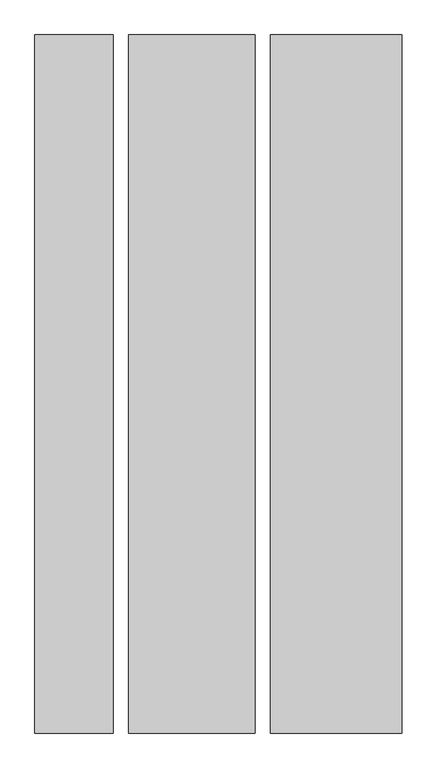
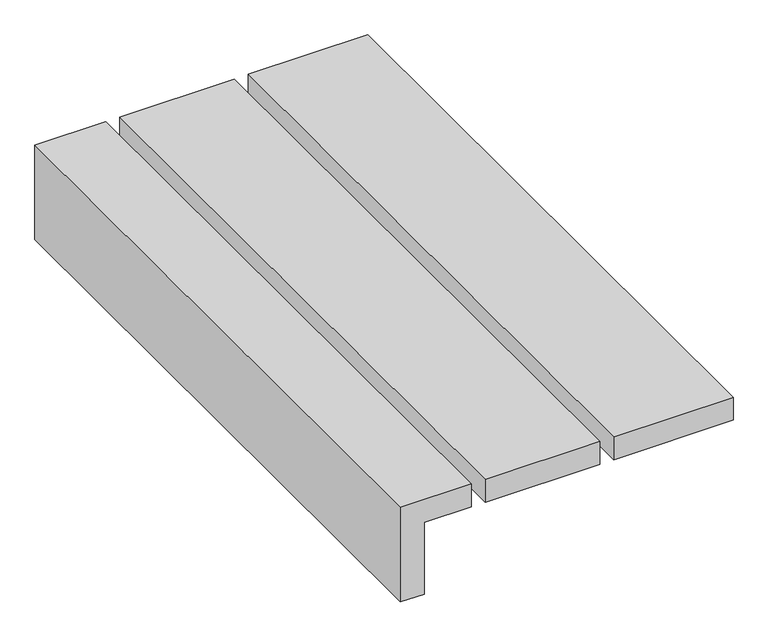
"""IFC4 building model written with IfcOpenShell, lengths in millimetres: proxy geometry, Blocking106 1:Blocking106 12412:297834 : Blocking106 1:Blocking106 12412:297834."""

from ifc_helpers import new_model, si_unit, frame, origin, place, context, project, spatial, polyline, outline, extrude, source, transform, mapped, element, save


def generic_models_f077f821(model_context):
    return source(origin(), model_context, "Body", "SweptSolid", [
        extrude(outline(polyline([(11504.1075575, 1225.4416475), (11504.1075575, -774.5583525), (11142.1575575, -774.5583525), (11142.1575575, 1225.4416475), (11504.1075575, 1225.4416475)])), frame((0.0, 0.0, 44042.7623529), z_axis=(0.0, 0.0, 1.0), x_axis=(1.0, 0.0, 0.0)), (0.0, 0.0, 1.0), 76.2),
        extrude(outline(polyline([(11926.3703128, 1225.4416475), (11926.3703128, -774.5583525), (11548.5575575, -774.5583525), (11548.5575575, 1225.4416475), (11926.3703128, 1225.4416475)])), frame((0.0, 0.0, 44042.7623529), z_axis=(0.0, 0.0, 1.0), x_axis=(1.0, 0.0, 0.0)), (0.0, 0.0, 1.0), 76.2),
        extrude(outline(polyline([(43803.0227817, 10949.6254643), (44042.7623529, 10949.6254643), (44042.7623529, 11097.7075575), (44118.9623529, 11097.7075575), (44118.9623529, 10873.4254643), (43803.0227817, 10873.4254643), (43803.0227817, 10949.6254643)])), frame((0.0, -774.5583525, 0.0), z_axis=(0.0, 1.0, 0.0), x_axis=(0.0, 0.0, 1.0)), (0.0, 0.0, 1.0), 2000.0),
    ])


if __name__ == "__main__":
    model = new_model("IFC4")
    model_context = context("Model", 3, world=origin())
    ifc_project = project(units=[si_unit("LENGTHUNIT", "METRE", prefix="MILLI")], contexts=[model_context])
    site = spatial("IfcSite", under=ifc_project)
    building = spatial("IfcBuilding", under=site)
    placement = place(None, origin())
    generic_models_shape = generic_models_f077f821(model_context)
    element("IfcBuildingElementProxy", 1, Name="Blocking106 1:Blocking106 12412:297834 : Blocking106 1:Blocking106 12412:297834", ObjectType="Blocking106 1:Blocking106 12412:297834 : Blocking106 1:Blocking106 12412:297834", at=placement, inside=building, context=model_context, shape_type="MappedRepresentation", body=[
        mapped(generic_models_shape, transform((0.0, 0.0, 0.0), x_axis=(1.0, 0.0, 0.0), y_axis=(0.0, 1.0, 0.0), z_axis=(0.0, 0.0, 1.0))),
    ])
    save(model, "model.ifc")

# Revit data of these elements
# Type "Blocking106 1:Blocking106 12412:297834 : Blocking106 1:Blocking106 12412:297834"
#   NameOverride = "Blocking106 1:Blocking106 12412:297834"
#   ObjectTypeOverride = "Blocking106 1:Blocking106 12412"
#   Reference = "Blocking106 12412"
#   Category = "Generic Models"
#   Tag = "297834"
# Element 1 (IfcBuildingElementProxy, "Blocking106 1:Blocking106 12412:297834 : Blocking106 1:Blocking106 12412:297834")
#   Materials on its faces: "POLYURETHANE SPRAY FOAM UNDER ROOF SUBSTRATE (SEE T-24 ENERGY REPORT FOR R-VALUE)"
# Materials
#   "POLYURETHANE SPRAY FOAM UNDER ROOF SUBSTRATE (SEE T-24 ENERGY REPORT FOR R-VALUE)": class "Unassigned", colour RGB 210 164 194, transparency 0, Cost = 0
